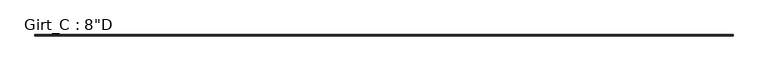
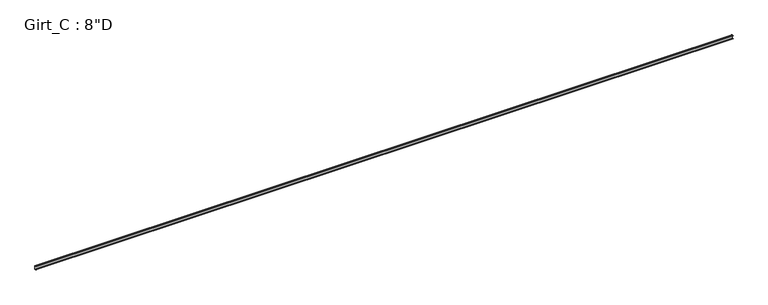
"""IFC4 building model written with IfcOpenShell, lengths in millimetres: beam geometry."""

from ifc_helpers import new_model, si_unit, point, frame, frame_2d, origin, place, context, project, spatial, polyline, circle_curve, trimmed, segment, composite_curve, outline, extrude, source, transform, mapped, element, save


def beam_b5f6ff4c(model_context):
    return source(origin(), model_context, "Body", "SweptSolid", [
        extrude(outline(composite_curve([segment(polyline([(-63.5, 101.6), (-3.3734375, 101.6)]), True, "CONTINUOUS"), segment(trimmed(circle_curve(frame_2d((-3.3734375, 96.8375)), 4.7625), [point((-3.3734375, 101.6))], [point((1.3890625, 96.8375))], False, "CARTESIAN"), True, "CONTINUOUS"), segment(polyline([(1.3890625, 96.8375), (1.3890625, -96.8375)]), True, "CONTINUOUS"), segment(trimmed(circle_curve(frame_2d((-3.3734375, -96.8375)), 4.7625), [point((1.3890625, -96.8375))], [point((-3.3734375, -101.6))], False, "CARTESIAN"), True, "CONTINUOUS"), segment(polyline([(-3.3734375, -101.6), (-63.5, -101.6), (-75.745104, -87.0068534), (-73.6169367, -85.221109), (-62.204539, -98.821875), (-3.2694106, -98.821875)]), True, "CONTINUOUS"), segment(trimmed(circle_curve(frame_2d((-3.3748024, -96.8389339)), 1.9857399), [point((-3.2694106, -98.821875))], [point((-1.3890625, -96.8389339))], True, "CARTESIAN"), True, "CONTINUOUS"), segment(polyline([(-1.3890625, -96.8389339), (-1.3890625, 96.8381931)]), True, "CONTINUOUS"), segment(trimmed(circle_curve(frame_2d((-3.3741066, 96.8381931)), 1.9850441), [point((-1.3890625, 96.8381931))], [point((-3.3005807, 98.821875))], True, "CARTESIAN"), True, "CONTINUOUS"), segment(polyline([(-3.3005807, 98.821875), (-62.204539, 98.821875), (-73.6169367, 85.221109), (-75.745104, 87.0068534), (-63.5, 101.6)]), True, "CONTINUOUS")], self_intersect=False)), frame((-20897.05625, 0.0, 0.0), z_axis=(1.0, 0.0, 0.0), x_axis=(0.0, 1.0, 0.0)), (0.0, 0.0, 1.0), 41949.6875),
    ])


if __name__ == "__main__":
    model = new_model("IFC4")
    model_context = context("Model", 3, world=origin())
    ifc_project = project(units=[si_unit("LENGTHUNIT", "METRE", prefix="MILLI")], contexts=[model_context])
    site = spatial("IfcSite", under=ifc_project)
    building = spatial("IfcBuilding", under=site)
    placement = place(None, origin())
    beam_shape = beam_b5f6ff4c(model_context)
    element("IfcBeam", 1, ObjectType="Girt_C : 8\"D", at=placement, inside=building, context=model_context, shape_type="MappedRepresentation", body=[
        mapped(beam_shape, transform((0.0, 0.0, 0.0), x_axis=(1.0, 0.0, 0.0), y_axis=(0.0, 1.0, 0.0), z_axis=(0.0, 0.0, 1.0))),
    ])
    save(model, "model.ifc")

# Revit data of these elements
# Type "Girt_C : 8\"D"
#   Web_Thickness = 0' - 0 7/64"
#   Length [instance default] = 10' - 0"
#   Leg_1 = 0' - 2 1/2"
#   Height = 0' - 8"
#   Structural Material [instance default] = none
# Element 1 (IfcBeam, "Girt_C : 8\"D")
#   Structural Material = Steel
#   Materials on its faces: "Steel"
# Materials
#   "Steel": class "Metal", colour RGB 118 118 114, transparency 0, Description = "Steel, mill finish", Cost = 0
